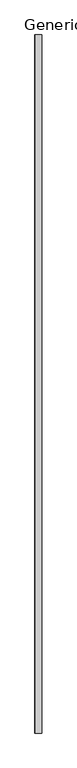
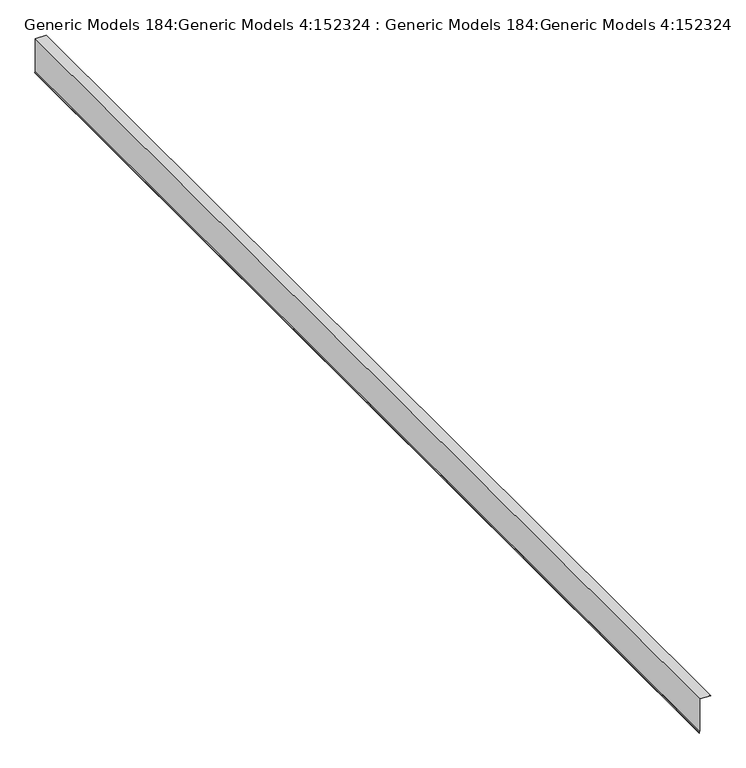
"""IFC4 building model written with IfcOpenShell, lengths in millimetres: proxy geometry, Generic Models 184:Generic Models 4:152324 : Generic Models 184:Generic Models 4:152324."""

from ifc_helpers import new_model, si_unit, frame, origin, place, context, project, spatial, polyline, outline, extrude, source, transform, mapped, element, save


def generic_models_184_generic_models_4_152324_generic_models_2daa7e4a(model_context):
    return source(origin(), model_context, "Body", "SweptSolid", [
        extrude(outline(polyline([(3073.9196249, -9478.8329326), (3633.6162181, -9478.8329326), (3626.1249529, -9299.042567), (3626.9180147, -9299.0095228), (3634.4437297, -9479.6266826), (3074.0595845, -9479.6266826), (3062.9658382, -9483.664476), (3047.9120757, -9483.664476), (3047.9120757, -9482.870726), (3062.8258787, -9482.870726), (3073.9196249, -9478.8329326)])), frame((0.0, -6674.7974793, 0.0), z_axis=(0.0, 1.0, 0.0), x_axis=(0.0, 0.0, 1.0)), (0.0, 0.0, 1.0), 18643.6),
    ])


if __name__ == "__main__":
    model = new_model("IFC4")
    model_context = context("Model", 3, world=origin())
    ifc_project = project(units=[si_unit("LENGTHUNIT", "METRE", prefix="MILLI")], contexts=[model_context])
    site = spatial("IfcSite", under=ifc_project)
    building = spatial("IfcBuilding", under=site)
    placement = place(None, origin())
    generic_models_184_generic_models_4_152324_generic_models_shape = generic_models_184_generic_models_4_152324_generic_models_2daa7e4a(model_context)
    element("IfcBuildingElementProxy", 1, Name="Generic Models 184:Generic Models 4:152324 : Generic Models 184:Generic Models 4:152324", ObjectType="Generic Models 184:Generic Models 4:152324 : Generic Models 184:Generic Models 4:152324", at=placement, inside=building, context=model_context, shape_type="MappedRepresentation", body=[
        mapped(generic_models_184_generic_models_4_152324_generic_models_shape, transform((0.0, 0.0, 0.0), x_axis=(1.0, 0.0, 0.0), y_axis=(0.0, 1.0, 0.0), z_axis=(0.0, 0.0, 1.0))),
    ])
    save(model, "model.ifc")

# Revit data of these elements
# Type "Generic Models 184:Generic Models 4:152324 : Generic Models 184:Generic Models 4:152324"
#   NameOverride = "Generic Models 184:Generic Models 4:152324"
#   ObjectTypeOverride = "Generic Models 184:Generic Models 4"
#   Reference = "Generic Models 4"
#   Category = "Generic Models"
#   Tag = "152324"
# Element 1 (IfcBuildingElementProxy, "Generic Models 184:Generic Models 4:152324 : Generic Models 184:Generic Models 4:152324")
#   Materials on its faces: "_(2) LAYERS NO. 30 ASTM D226 ASPHALT SATURATED ORGANIC FELT 997"
# Materials
#   "_(2) LAYERS NO. 30 ASTM D226 ASPHALT SATURATED ORGANIC FELT 997": class "Unassigned", colour RGB 67 154 161, transparency 0
